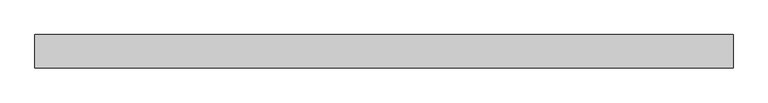
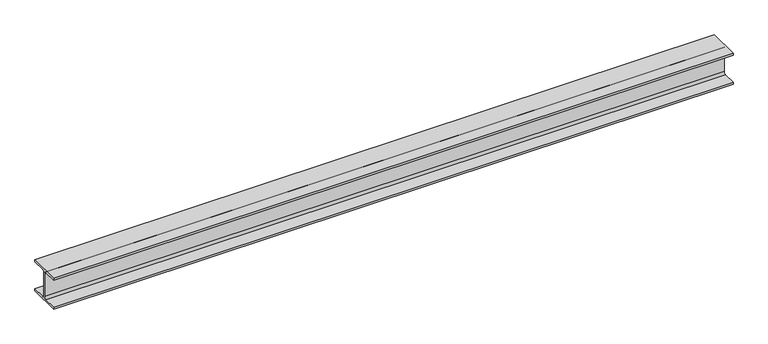
"""IFC4 building model written with IfcOpenShell, lengths in millimetres: beam geometry, 0912_Steel Framing_H-KSD3502 : H_SB_ASB_H-200x200x8x12."""

from ifc_helpers import new_model, si_unit, point, frame, frame_2d, origin, place, context, project, spatial, polyline, circle_curve, trimmed, segment, composite_curve, outline, extrude, source, transform, mapped, element, save


def beam_301e8018(model_context):
    return source(origin(), model_context, "Body", "SweptSolid", [
        extrude(outline(composite_curve([segment(polyline([(100.0, -88.0), (100.0, -100.0), (-100.0, -100.0), (-100.0, -88.0), (-17.0, -88.0)]), True, "CONTINUOUS"), segment(trimmed(circle_curve(frame_2d((-17.0, -75.0)), 13.0), [point((-17.0, -88.0))], [point((-4.0, -75.0))], True, "CARTESIAN"), True, "CONTINUOUS"), segment(polyline([(-4.0, -75.0), (-4.0, 75.0)]), True, "CONTINUOUS"), segment(trimmed(circle_curve(frame_2d((-17.0, 75.0)), 13.0), [point((-4.0, 75.0))], [point((-17.0, 88.0))], True, "CARTESIAN"), True, "CONTINUOUS"), segment(polyline([(-17.0, 88.0), (-100.0, 88.0), (-100.0, 100.0), (100.0, 100.0), (100.0, 88.0), (17.0, 88.0)]), True, "CONTINUOUS"), segment(trimmed(circle_curve(frame_2d((17.0, 75.0)), 13.0), [point((17.0, 88.0))], [point((4.0, 75.0))], True, "CARTESIAN"), True, "CONTINUOUS"), segment(polyline([(4.0, 75.0), (4.0, -75.0)]), True, "CONTINUOUS"), segment(trimmed(circle_curve(frame_2d((17.0, -75.0)), 13.0), [point((4.0, -75.0))], [point((17.0, -88.0))], True, "CARTESIAN"), True, "CONTINUOUS"), segment(polyline([(17.0, -88.0), (100.0, -88.0)]), True, "CONTINUOUS")], self_intersect=False)), frame((-2029.7220739, 0.0, 0.0), z_axis=(1.0, 0.0, 0.0), x_axis=(0.0, 1.0, 0.0)), (0.0, 0.0, 1.0), 4201.2459651),
    ])


if __name__ == "__main__":
    model = new_model("IFC4")
    model_context = context("Model", 3, world=origin())
    ifc_project = project(units=[si_unit("LENGTHUNIT", "METRE", prefix="MILLI")], contexts=[model_context])
    site = spatial("IfcSite", under=ifc_project)
    building = spatial("IfcBuilding", under=site)
    placement = place(None, origin())
    beam_shape = beam_301e8018(model_context)
    element("IfcBeam", 1, ObjectType="0912_Steel Framing_H-KSD3502 : H_SB_ASB_H-200x200x8x12", at=placement, inside=building, context=model_context, shape_type="MappedRepresentation", body=[
        mapped(beam_shape, transform((0.0, 0.0, 0.0), x_axis=(1.0, 0.0, 0.0), y_axis=(0.0, 1.0, 0.0), z_axis=(0.0, 0.0, 1.0))),
    ])
    save(model, "model.ifc")

# Revit data of these elements
# Type "0912_Steel Framing_H-KSD3502 : H_SB_ASB_H-200x200x8x12"
#   H_WM Code_1 = "S01AA002-00001 | Main Steel Structure Fabrication Work | Shelter/Building | Medium Steel - Standard (90KG/M>Weight≥30KG/M) | Material: (   )"
#   H_WM Code_2 = "S03AA028-00001 | Main Steel Structure Erection Work | Shelter/Building | Medium Steel (90KG/M>Weight≥30KG/M) | Material: (   )"
#   H_WM Code_3 = "S01AA010-00001 | Main Steel Structure Fabrication Work | Shelter/Building | Steel Painting/Coating | for Non-Fireproofed Steel Surface, Surface Preparation, Primer, Second & Final Coat | Material: (   )"
#   H_Q'ty Cal Type Tag = "SB-Q2"
#   Width = 20.0 cm
#   Web Thickness = 0.8 cm
#   Web Fillet = 1.3 cm
#   Warping Constant = 141000.0 cm⁶
#   W = 0
#   Torsional Moment of Inertia = 26.2485 cm⁴
#   Section Area = 63.53 cm²
#   Plastic Modulus weak axis = 244.0 cm³
#   Plastic Modulus strong axis = 525.0 cm³
#   Perimeter = 1.16 m²/m
#   Nominal Weight = 49.90 kgf/m
#   Moment of Inertia weak axis = 1600.00 cm⁴
#   Moment of Inertia strong axis = 4720.00 cm⁴
#   Height = 20.0 cm
#   Flange Thickness = 1.2 cm
#   Elastic Modulus weak axis = 160.0 cm³
#   Elastic Modulus strong axis = 472.0 cm³
#   Centroid Vertical = 10.0 cm
#   Centroid Horizontal = 10.0 cm
#   Ix = 47200000
#   Length [instance default] = 1.5240 m
#   Zx = 525000
#   b = 0.2000 m
#   h = 0.2000 m
#   r = 0.0130 m
#   s = 0.0080 m
#   t = 0.0120 m
#   A = 0.006353 m²
#   Structural Material [instance default] = Steel, 45-345
#   Assembly Code = ""
# Element 1 (IfcBeam, "0912_Steel Framing_H-KSD3502 : H_SB_ASB_H-200x200x8x12")
#   Structural Material = none
# Materials
#   "Steel, 45-345": class "Metal", colour RGB 189 187 185, transparency 0, Description = "Steel 345 MPa", Cost = 0
